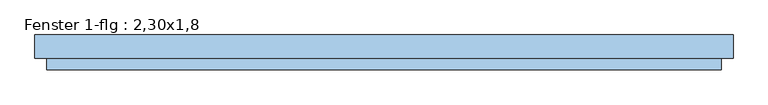
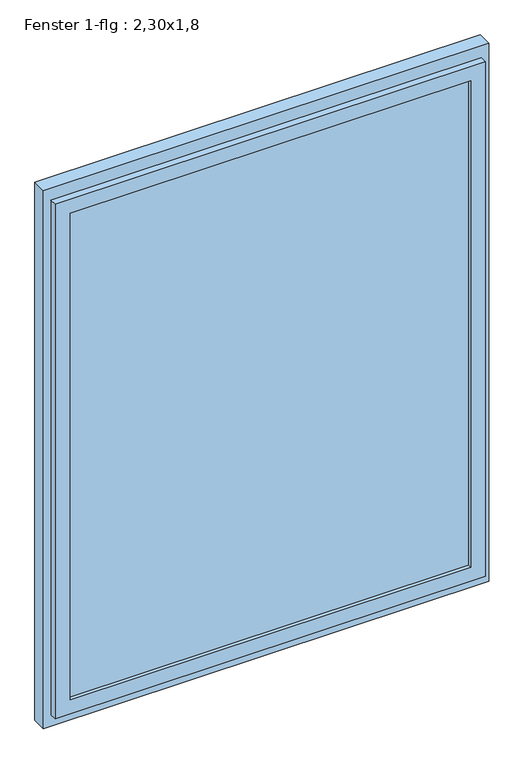
"""IFC4 building model written with IfcOpenShell, lengths in millimetres: window geometry, Fenster 1-flg : 2,30x1,8."""

from ifc_helpers import new_model, si_unit, frame, origin, place, context, project, spatial, polyline, outline, extrude, faceted_brep, source, transform, mapped, element, save


def fenster_1_flg_2_30x1_8_d6f49dcb(model_context):
    return source(origin(), model_context, "Body", "SolidModel", [
        extrude(outline(polyline([(3300.0, 900.0), (3300.0, -900.0), (1000.0, -900.0), (1000.0, 900.0), (3300.0, 900.0)]), holes=[polyline([(3220.0, 840.0), (1080.0, 840.0), (1080.0, -840.0), (3220.0, -840.0), (3220.0, 840.0)])]), frame((0.0, -55.0, 0.0), z_axis=(0.0, 1.0, 0.0), x_axis=(0.0, 0.0, 1.0)), (0.0, 0.0, 1.0), 60.0),
        faceted_brep([(870.0, -55.0, 3250.0), (870.0, -85.0, 3250.0), (870.0, -85.0, 1050.0), (870.0, -55.0, 1050.0), (-870.0, -85.0, 3250.0), (-870.0, -85.0, 1050.0), (810.0, -85.0, 1110.0), (-810.0, -85.0, 1110.0), (-810.0, -85.0, 3190.0), (810.0, -85.0, 3190.0), (-870.0, -55.0, 1050.0), (-870.0, -55.0, 3250.0), (840.0, -55.0, 3220.0), (-840.0, -55.0, 3220.0), (-840.0, -55.0, 1080.0), (840.0, -55.0, 1080.0), (840.0, -25.0, 3220.0), (840.0, -25.0, 1080.0), (-840.0, -25.0, 1080.0), (-840.0, -25.0, 3220.0), (810.0, -25.0, 3190.0), (-810.0, -25.0, 3190.0), (-810.0, -25.0, 1110.0), (810.0, -25.0, 1110.0)], [[[0, 1, 2, 3]], [[1, 4, 5, 2], [6, 7, 8, 9]], [[3, 2, 5, 10]], [[3, 10, 11, 0], [12, 13, 14, 15]], [[16, 12, 15, 17]], [[17, 15, 14, 18]], [[17, 18, 19, 16], [20, 21, 22, 23]], [[9, 20, 23, 6]], [[6, 23, 22, 7]], [[10, 5, 4, 11]], [[18, 14, 13, 19]], [[7, 22, 21, 8]], [[11, 4, 1, 0]], [[19, 13, 12, 16]], [[8, 21, 20, 9]]]),
        extrude(outline(polyline([(810.0, -70.0), (-810.0, -70.0), (-810.0, -40.0), (810.0, -40.0), (810.0, -70.0)])), frame((0.0, 0.0, 1110.0), z_axis=(0.0, 0.0, 1.0), x_axis=(1.0, 0.0, 0.0)), (0.0, 0.0, 1.0), 2080.0),
    ])


if __name__ == "__main__":
    model = new_model("IFC4")
    model_context = context("Model", 3, world=origin())
    ifc_project = project(units=[si_unit("LENGTHUNIT", "METRE", prefix="MILLI")], contexts=[model_context])
    site = spatial("IfcSite", under=ifc_project)
    building = spatial("IfcBuilding", under=site)
    placement = place(None, origin())
    fenster_1_flg_2_30x1_8_shape = fenster_1_flg_2_30x1_8_d6f49dcb(model_context)
    element("IfcWindow", 1, ObjectType="Fenster 1-flg : 2,30x1,8", at=placement, inside=building, context=model_context, shape_type="MappedRepresentation", body=[
        mapped(fenster_1_flg_2_30x1_8_shape, transform((0.0, 0.0, 0.0), x_axis=(1.0, 0.0, 0.0), y_axis=(0.0, 1.0, 0.0), z_axis=(0.0, 0.0, 1.0))),
    ])
    save(model, "model.ifc")

# Revit data of these elements
# Type "Fenster 1-flg : 2,30x1,8"
#   Type Mark = "71"
#   Operation = "SinglePanel"
#   Keynote = "16.05.01"
#   Visual Light Transmittance = 0.9
#   Solar Heat Gain Coefficient = 0.86
#   Rough Width = 1.800 m
#   Rough Height = 2.300 m
#   Heat Transfer Coefficient (U) = 5.5617 W/(m²·K)
#   Rahmentiefe = 0.060 m
#   Rahmenhöhe - unten = 0.080 m
#   Rahmenhöhe - oben = 0.080 m
#   Rahmenbreite = 0.060 m
#   Height = 2.300 m
#   Tiefe Flügel = 0.060 m
#   Flügelbreite = 0.060 m
#   Einbautiefe (von außen) [instance default] = 0.100 m
#   Width = 1.800 m
#   Klappflügel [instance default] = no
#   Kippflügel [instance default] = yes
#   Öffnungsrichtung in Draufsicht anzeigen [instance default] = no
#   Drehflügel 1 [instance default] = yes
#   Rahmen 1 [instance default] = none
#   Glas [instance default] = none
#   Flügel [instance default] = none
#   Fensterbank Innenseite [instance default] = none
#   Fensterbank Außenseite [instance default] = none
#   Construction Type Id = ""
#   Wall Closure = (empty or 0)
#   Analytic Construction = (empty or 0)
# Element 1 (IfcWindow, "Fenster 1-flg : 2,30x1,8")
#   Einbautiefe (von außen) = 0.220 m
#   Materials on its faces: "Kunststoff - Weiß", "Glas"
# Materials
#   "Kunststoff - Weiß": class "Kunststoff", colour RGB 249 249 249, transparency 0, Cost = 0
#   "Glas": class "Glas", colour RGB 0 0 255, transparency 0.75, Comments = "Render-Darstellung nicht aktualisiert ", Cost = 0
